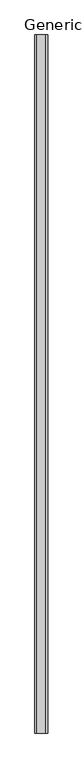
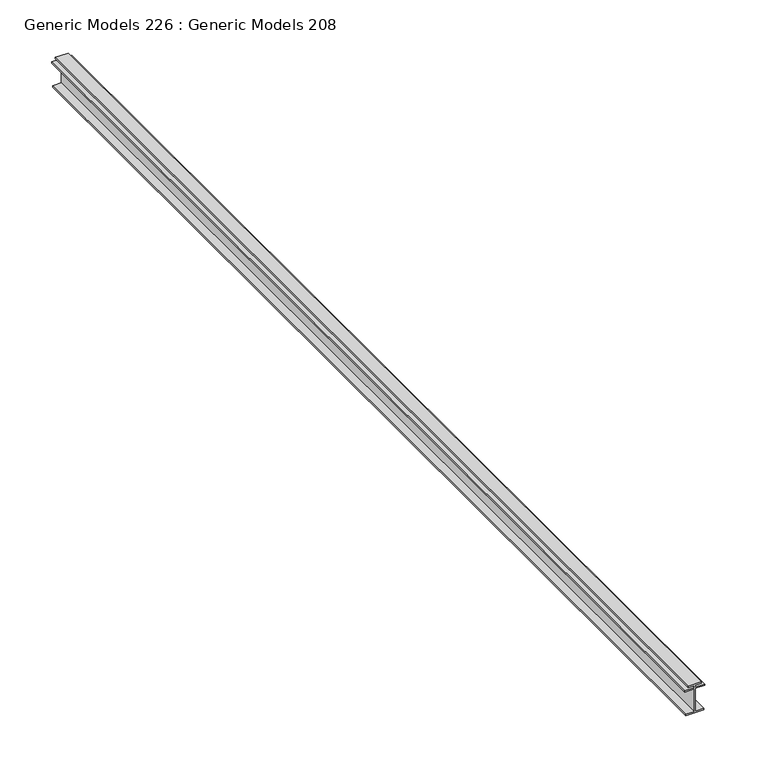
"""IFC4 building model written with IfcOpenShell, lengths in millimetres: proxy geometry, Generic Models 226 : Generic Models 208."""

from ifc_helpers import new_model, si_unit, frame, origin, place, context, project, spatial, polyline, outline, extrude, source, transform, mapped, element, save


def generic_models_226_generic_models_208_a943e66d(model_context):
    return source(origin(), model_context, "Body", "SweptSolid", [
        extrude(outline(polyline([(2164.159375, 54429.8292403), (2164.159375, 54440.1142176), (2137.4318993, 54440.1142176), (2137.4318993, 54430.7344915), (2135.8443993, 54430.7344915), (2135.8443993, 54450.7934243), (2137.4318993, 54450.7934243), (2137.4318993, 54441.7017176), (2164.159375, 54441.7017176), (2164.159375, 54451.986695), (2165.746875, 54451.986695), (2165.746875, 54441.7017176), (2168.128125, 54441.7017176), (2168.128125, 54448.0517176), (2169.715625, 54448.0517176), (2169.715625, 54433.4761981), (2168.128125, 54433.4761981), (2168.128125, 54440.1142176), (2165.746875, 54440.1142176), (2165.746875, 54429.8292403), (2164.159375, 54429.8292403)])), frame((0.0, -228.7033818, 0.0), z_axis=(0.0, 1.0, 0.0), x_axis=(0.0, 0.0, 1.0)), (0.0, 0.0, 1.0), 1219.2),
    ])


if __name__ == "__main__":
    model = new_model("IFC4")
    model_context = context("Model", 3, world=origin())
    ifc_project = project(units=[si_unit("LENGTHUNIT", "METRE", prefix="MILLI")], contexts=[model_context])
    site = spatial("IfcSite", under=ifc_project)
    building = spatial("IfcBuilding", under=site)
    placement = place(None, origin())
    generic_models_226_generic_models_208_shape = generic_models_226_generic_models_208_a943e66d(model_context)
    element("IfcBuildingElementProxy", 1, Name="Generic Models 226 : Generic Models 208", ObjectType="Generic Models 226 : Generic Models 208", at=placement, inside=building, context=model_context, shape_type="MappedRepresentation", body=[
        mapped(generic_models_226_generic_models_208_shape, transform((0.0, 0.0, 0.0), x_axis=(1.0, 0.0, 0.0), y_axis=(0.0, 1.0, 0.0), z_axis=(0.0, 0.0, 1.0))),
    ])
    save(model, "model.ifc")
